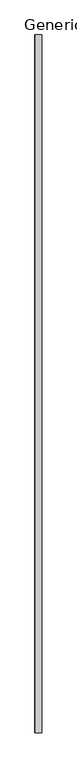
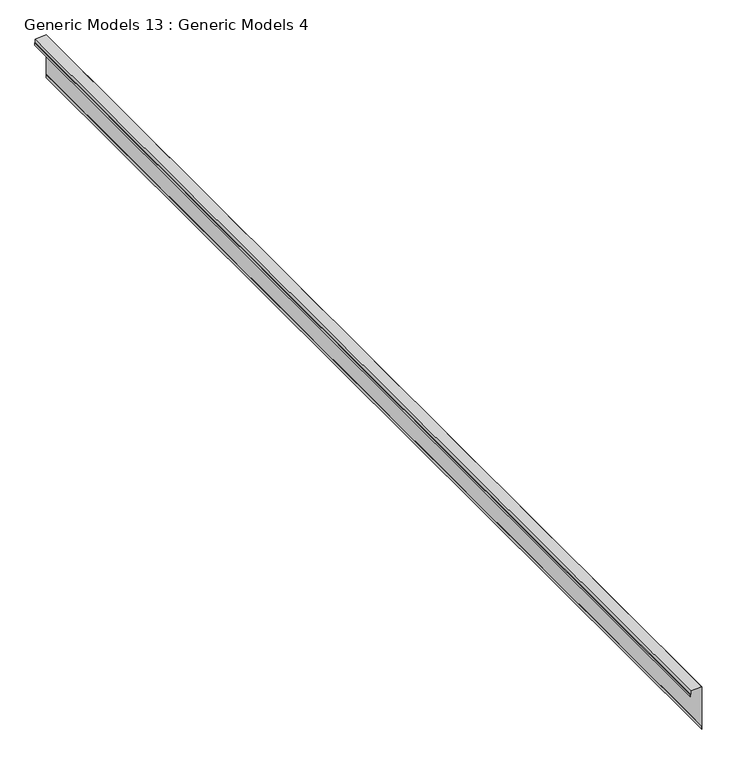
"""IFC4 building model written with IfcOpenShell, lengths in millimetres: proxy geometry, Generic Models 13 : Generic Models 4."""

from ifc_helpers import new_model, si_unit, frame, origin, place, context, project, spatial, polyline, outline, extrude, source, transform, mapped, element, save


def generic_models_13_generic_models_4_df24dfde(model_context):
    return source(origin(), model_context, "Body", "SweptSolid", [
        extrude(outline(polyline([(127013.3250789, 8389.1524314), (127020.4570194, 8391.7482454), (127078.1640881, 8391.7482454), (127085.7438493, 8573.6625161), (126401.732454, 8573.6625161), (126392.819518, 8576.9065595), (126345.7971943, 8576.9065595), (126345.7971943, 8577.7003095), (126393.3203108, 8577.7003095), (126402.2332468, 8574.4562661), (127086.571361, 8574.4562661), (127078.9254539, 8390.9544954), (127020.596979, 8390.9544954), (127013.4650384, 8388.3586814), (126974.0744351, 8388.3586814), (126974.0744351, 8389.1524314), (127013.3250789, 8389.1524314)])), frame((0.0, -6864.9230338, 0.0), z_axis=(0.0, 1.0, 0.0), x_axis=(0.0, 0.0, 1.0)), (0.0, 0.0, 1.0), 18643.6),
    ])


if __name__ == "__main__":
    model = new_model("IFC4")
    model_context = context("Model", 3, world=origin())
    ifc_project = project(units=[si_unit("LENGTHUNIT", "METRE", prefix="MILLI")], contexts=[model_context])
    site = spatial("IfcSite", under=ifc_project)
    building = spatial("IfcBuilding", under=site)
    placement = place(None, origin())
    generic_models_13_generic_models_4_shape = generic_models_13_generic_models_4_df24dfde(model_context)
    element("IfcBuildingElementProxy", 1, Name="Generic Models 13 : Generic Models 4", ObjectType="Generic Models 13 : Generic Models 4", at=placement, inside=building, context=model_context, shape_type="MappedRepresentation", body=[
        mapped(generic_models_13_generic_models_4_shape, transform((0.0, 0.0, 0.0), x_axis=(1.0, 0.0, 0.0), y_axis=(0.0, 1.0, 0.0), z_axis=(0.0, 0.0, 1.0))),
    ])
    save(model, "model.ifc")

# Revit data of these elements
# Element 1 (IfcBuildingElementProxy, "Generic Models 13 : Generic Models 4")
#   Materials on its faces: "_(2) LAYERS NO. 30 ASTM D226 ASPHALT SATURATED ORGANIC FELT"
# Materials
#   "_(2) LAYERS NO. 30 ASTM D226 ASPHALT SATURATED ORGANIC FELT": class "Generic", colour RGB 67 154 161, transparency 0, Cost = 0
